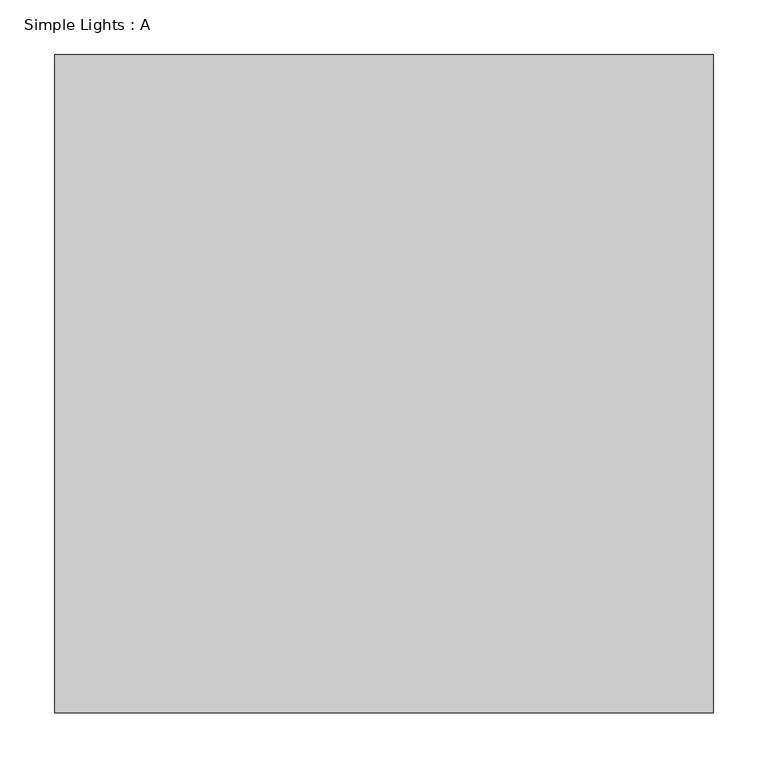
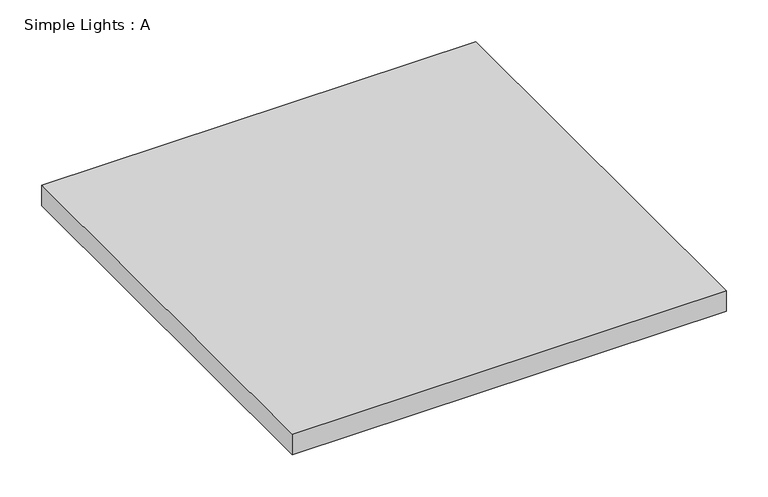
"""IFC4 building model written with IfcOpenShell, lengths in millimetres: light fixture geometry, Simple Lights : A."""

from ifc_helpers import new_model, si_unit, frame, origin, place, context, project, spatial, polyline, outline, extrude, source, transform, mapped, element, save


def simple_lights_a_61f39cf9(model_context):
    return source(origin(), model_context, "Body", "SweptSolid", [
        extrude(outline(polyline([(300.0, 300.0), (300.0, -300.0), (-300.0, -300.0), (-300.0, 300.0), (300.0, 300.0)])), frame((0.0, 0.0, -30.0), z_axis=(0.0, 0.0, 1.0), x_axis=(1.0, 0.0, 0.0)), (0.0, 0.0, 1.0), 30.0),
    ])


if __name__ == "__main__":
    model = new_model("IFC4")
    model_context = context("Model", 3, world=origin())
    ifc_project = project(units=[si_unit("LENGTHUNIT", "METRE", prefix="MILLI")], contexts=[model_context])
    site = spatial("IfcSite", under=ifc_project)
    building = spatial("IfcBuilding", under=site)
    placement = place(None, origin())
    simple_lights_a_shape = simple_lights_a_61f39cf9(model_context)
    element("IfcLightFixture", 1, ObjectType="Simple Lights : A", at=placement, inside=building, context=model_context, shape_type="MappedRepresentation", body=[
        mapped(simple_lights_a_shape, transform((0.0, 0.0, 0.0), x_axis=(1.0, 0.0, 0.0), y_axis=(0.0, 1.0, 0.0), z_axis=(0.0, 0.0, 1.0))),
    ])
    save(model, "model.ifc")

# Revit data of these elements
# Type "Simple Lights : A"
#   B = no
#   A = yes
#   Default Elevation = 0
